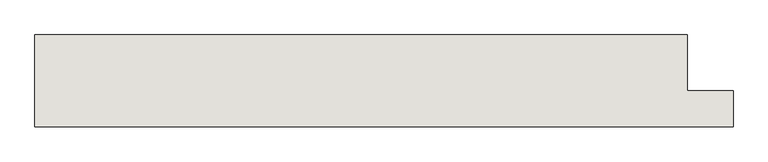
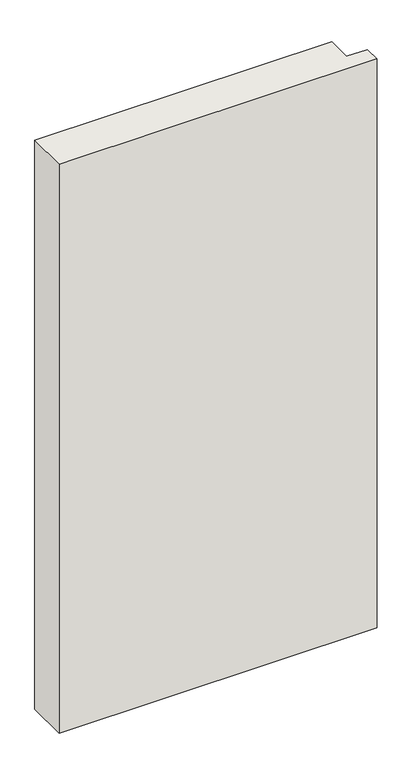
"""IFC4 building model written with IfcOpenShell, lengths in millimetres: wall geometry, Holzwand."""

from ifc_helpers import new_model, si_unit, origin, origin_with_axes, place, context, project, spatial, polyline, outline, extrude, source, transform, mapped, element, save


def wall_00aa1bb1(model_context):
    return source(origin(), model_context, "Body", "SweptSolid", [
        extrude(outline(polyline([(1524.0204176, 0.0), (0.0, 0.0), (0.0, 200.0), (1424.0204176, 200.0), (1424.0204176, 78.0), (1524.0204176, 78.0), (1524.0204176, 0.0)])), origin_with_axes(), (0.0, 0.0, 1.0), 2880.0),
    ])


if __name__ == "__main__":
    model = new_model("IFC4")
    model_context = context("Model", 3, world=origin())
    ifc_project = project(units=[si_unit("LENGTHUNIT", "METRE", prefix="MILLI")], contexts=[model_context])
    site = spatial("IfcSite", under=ifc_project)
    building = spatial("IfcBuilding", under=site)
    placement = place(None, origin())
    wall_shape = wall_00aa1bb1(model_context)
    element("IfcWall", 1, ObjectType="Holzwand", at=placement, inside=building, context=model_context, shape_type="MappedRepresentation", body=[
        mapped(wall_shape, transform((0.0, 0.0, 0.0), x_axis=(1.0, 0.0, 0.0), y_axis=(0.0, 1.0, 0.0), z_axis=(0.0, 0.0, 1.0))),
    ])
    save(model, "model.ifc")

# Revit data of these elements
# Project information
#   Organization Name = "Organization Name"
#   Organization Description = "Organization Description"
#   Building Name = "Building Name"
#   IfcOrganization = "KURIARCHITEKTEN"
#   IfcApplicationVersion = "2024.1"
#   IfcApplicationName = "Allplan"
#   IfcSite GUID = "3xMs$kp1n46ejeur8tozco"
#   IfcBuilding GUID = "0i8UyhEYT3nv9HLlo1H2X7"
#   IfcProject GUID = "2x1YFttxr4OvBiL8xtaqeA"
#   IfcDecomposes = "BVH Tammik Wohnhaus Waldrain"
#   IfcDecomposesGUID = "2x1YFttxr4OvBiL8xtaqeA"
#   IfcPropertySetList = "\"AllplanAttributes\""
#   BuildingName = "WALDRAIN"
#   SiteName = "BAUANTRAG"
#   IfcProject Name = "BVH Tammik Wohnhaus Waldrain"
#   AllplanAttributes.Land = "IFC - Land"
#   AllplanAttributes.Bundesland = "IFC - Bundesland"
#   AllplanAttributes.Prüfer = "Prüfstatiker"
#   AllplanAttributes.Bauherr = "Jeremy Tammik"
#   AllplanAttributes.Bruttogeschossfläche = "IFC - Bruttogeschossfläche"
#   AllplanAttributes.Projektleiter = "Projektleitername"
#   AllplanAttributes.Architekt = "Architektenname"
#   AllplanAttributes.Statik = "Statiker"
#   AllplanAttributes.Elektro = "Elektroplaner"
#   AllplanAttributes.Heizung = "Heizungsplaner"
#   AllplanAttributes.Sanitär = "Sanitärplaner"
#   AllplanAttributes.Bebaubare Fläche = "IFC - bebaubare Fläche"
#   AllplanAttributes.Maximale Gebäudehöhe = "IFC - Maximale Gebäudehöhe"
#   AllplanAttributes.Bruttogrundstücksfläche = "IFC - Bruttogrundstücksfläche"
#   AllplanAttributes.Normalhöhennull = "IFC - Höhe über NN"
#   AllplanAttributes.Projektvorlage = "IBD 2023"
#   AllplanAttributes.Bauvorhaben = "Neubau eines Wohnhauses mit gemeinschaftlich nutzbaren Wohneinheiten"
#   AllplanAttributes.Bauherr Straße = "Mühlesteig 7"
#   AllplanAttributes.Bauherr Plz/Ort = "CH-4102 Binningen"
#   AllplanAttributes.Architekt Straße = "Architektenstrasse 111"
#   AllplanAttributes.Architekt Plz/Ort = "72108 Architektenort"
#   AllplanAttributes.Bauvorhaben Straße = "Sonnenweg 6"
#   AllplanAttributes.Bauvorhaben Plz/Ort = "79539 Lörrach"
#   AllplanAttributes.Projektnummer = "2023"
#   AllplanAttributes.Architekt Telefonnummer = "07472-93791-0"
#   AllplanAttributes.Architekt Telefaxnummer = "07472/93791-29"
#   AllplanAttributes.Projektbeschreibung = "Projektnamen Ergänzung"
#   AllplanAttributes.Geographische Länge = "IFC - Geografische Länge"
#   AllplanAttributes.Geographische Breite = "IFC - Geografische Breite"
#   AllplanAttributes.Architekt E-Mail = "Architekt@email.de"
#   Original IFC File Name = "Y:\\j\\doc\\house\\huenerberg\\waldrain\\html\\waldrain.github.io\\doc\\biz\\kuri\\2024-09-25\\0_3d.ifc"
#   Original IFC File Size = "6299888"
#   Revit File Last Updated = "638628552499634221"
#   Revit Importer Version = "Importer 25.0.2.419"
#   Import Method = "Hybrid"
#   Project Issue Date = "Issue Date"
#   Project Status = "Project Status"
#   Client Name = "Client Name"
#   Project Address = "Enter address here\nAddress Line 2"
#   Project Name = "Project Name"
#   Project Number = "Project Number"
# Element 1 (IfcWall, "Holzwand")
#   Materials on its faces: "holzschalung"
# Materials
#   "holzschalung": class "Unassigned", colour RGB 128 128 128, transparency 0
